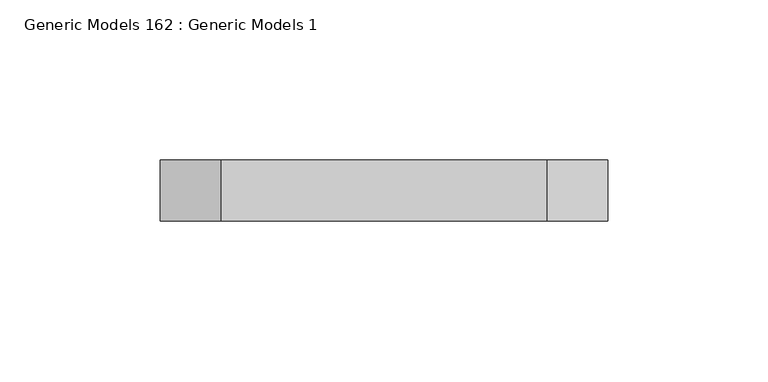
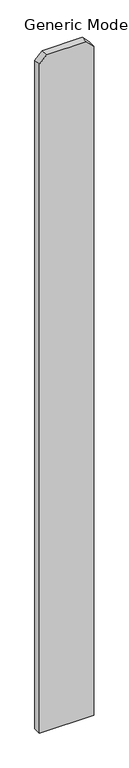
"""IFC4 building model written with IfcOpenShell, lengths in millimetres: proxy geometry, Generic Models 162 : Generic Models 1."""

import ifcopenshell
import ifcopenshell.guid

model = None  # the IFC model being written
_history = None  # IfcOwnerHistory: only IFC2X3 demands one
_inside = {}  # id of a spatial element -> (the spatial element, [elements in it])
_under = {}  # id of a project, library or spatial element -> (it, [spatial elements below it])
_declared = {}  # id of a project -> (the project, [libraries it declares])
_typed = {}  # id of a type object -> (the type object, [elements of that type])
_made_of = {}  # id of a material, layer set ... -> (it, [elements and type objects made of it])


def new_model(schema):
    """Start an empty IFC model of exactly this schema.

    Asked for "IFC4X3", IfcOpenShell would pick the latest addendum, in which some entities
    have other attributes; the version numbers below select the first issue.
    IFC2X3 requires an IfcOwnerHistory on every rooted entity: one is made here for all.
    """
    global model, _history
    if schema == "IFC4X3":
        model = ifcopenshell.file(schema_version=(4, 3, 0, 0))
    else:
        model = ifcopenshell.file(schema=schema)
    _inside.clear()
    _under.clear()
    _declared.clear()
    _typed.clear()
    _made_of.clear()
    _history = None
    if model.schema == "IFC2X3":
        org = make("IfcOrganization", Name="unknown")
        user = make(
            "IfcPersonAndOrganization",
            ThePerson=make("IfcPerson", FamilyName="unknown"),
            TheOrganization=org,
        )
        app = make(
            "IfcApplication",
            ApplicationDeveloper=org,
            Version="unknown",
            ApplicationFullName="unknown",
            ApplicationIdentifier="unknown",
        )
        _history = make(
            "IfcOwnerHistory",
            OwningUser=user,
            OwningApplication=app,
            ChangeAction="ADDED",
            CreationDate=0,
        )
    return model


def make(cls, **values):
    """One entity of the class cls with the attributes given. An attribute that is None is left unset."""
    return model.create_entity(
        cls, **{name: value for name, value in values.items() if value is not None}
    )


def rooted(cls, **values):
    """An entity with a GlobalId (a new one), such as an element, a storey or a relation."""
    return make(cls, GlobalId=ifcopenshell.guid.new(), OwnerHistory=_history, **values)


def si_unit(unit_type, name, prefix=None):
    """IfcSIUnit, for example si_unit("LENGTHUNIT", "METRE", prefix="MILLI")."""
    return make("IfcSIUnit", UnitType=unit_type, Prefix=prefix, Name=name)


def assignment(units):
    """IfcUnitAssignment: the units of a project."""
    return None if units is None else make("IfcUnitAssignment", Units=units)


def point(xyz):
    """IfcCartesianPoint."""
    return None if xyz is None else make("IfcCartesianPoint", Coordinates=xyz)


def direction(xyz):
    """IfcDirection."""
    return None if xyz is None else make("IfcDirection", DirectionRatios=xyz)


def frame(location, z_axis=None, x_axis=None):
    """IfcAxis2Placement3D, a coordinate frame: its origin and axes. An axis left out is left unset."""
    return make(
        "IfcAxis2Placement3D",
        Location=point(location),
        Axis=direction(z_axis),
        RefDirection=direction(x_axis),
    )


def origin():
    """The frame at (0, 0, 0) with its axes left unset."""
    return frame((0.0, 0.0, 0.0))


def place(relative_to, where):
    """IfcLocalPlacement: puts the frame where relative to a parent placement (None: the world)."""
    return make(
        "IfcLocalPlacement", PlacementRelTo=relative_to, RelativePlacement=where
    )


def context(
    kind, dimensions, precision=None, world=None, true_north=None, identifier=None
):
    """IfcGeometricRepresentationContext, for example the 3D "Model" context."""
    return make(
        "IfcGeometricRepresentationContext",
        ContextIdentifier=identifier,
        ContextType=kind,
        CoordinateSpaceDimension=dimensions,
        Precision=precision,
        WorldCoordinateSystem=world,
        TrueNorth=true_north,
    )


def project(units=None, contexts=None):
    """IfcProject with its units and contexts."""
    return rooted(
        "IfcProject",
        Name="project",
        RepresentationContexts=contexts,
        UnitsInContext=assignment(units),
    )


def spatial(cls, under=None, at=None, **own):
    """A site, building, storey or space (cls), placed at a placement, below another one or the project."""
    s = rooted(cls, ObjectPlacement=at, **own)
    if under is not None:
        _under.setdefault(under.id(), (under, []))[1].append(s)
    return s


def polyline(points):
    """IfcPolyline through the points."""
    return make("IfcPolyline", Points=[point(p) for p in points])


def outline(outer, holes=None, kind="AREA"):
    """IfcArbitraryClosedProfileDef: a profile drawn as a closed curve; with holes, ...WithVoids."""
    if holes is None:
        return make("IfcArbitraryClosedProfileDef", ProfileType=kind, OuterCurve=outer)
    return make(
        "IfcArbitraryProfileDefWithVoids",
        ProfileType=kind,
        OuterCurve=outer,
        InnerCurves=holes,
    )


def extrude(swept, where, along, depth):
    """IfcExtrudedAreaSolid: the profile swept, set in the frame where, extruded along a direction by depth."""
    return make(
        "IfcExtrudedAreaSolid",
        SweptArea=swept,
        Position=where,
        ExtrudedDirection=direction(along),
        Depth=depth,
    )


def shape(context_of_items, identifier, shape_type, items):
    """IfcShapeRepresentation: the items that make up one representation, for example the "Body"."""
    return make(
        "IfcShapeRepresentation",
        ContextOfItems=context_of_items,
        RepresentationIdentifier=identifier,
        RepresentationType=shape_type,
        Items=items,
    )


def source(mapping_origin, context_of_items, identifier, shape_type, items):
    """IfcRepresentationMap: a shape defined once, which mapped items show again and again."""
    return make(
        "IfcRepresentationMap",
        MappingOrigin=mapping_origin,
        MappedRepresentation=shape(context_of_items, identifier, shape_type, items),
    )


def transform(
    local_origin,
    x_axis=None,
    y_axis=None,
    z_axis=None,
    scale=None,
    scale2=None,
    scale3=None,
    uniform=True,
):
    """IfcCartesianTransformationOperator3D, or its non-uniform kind. x_axis, y_axis, z_axis: its Axis1, 2, 3."""
    if uniform:
        return make(
            "IfcCartesianTransformationOperator3D",
            Axis1=direction(x_axis),
            Axis2=direction(y_axis),
            LocalOrigin=point(local_origin),
            Scale=scale,
            Axis3=direction(z_axis),
        )
    return make(
        "IfcCartesianTransformationOperator3DnonUniform",
        Axis1=direction(x_axis),
        Axis2=direction(y_axis),
        LocalOrigin=point(local_origin),
        Scale=scale,
        Axis3=direction(z_axis),
        Scale2=scale2,
        Scale3=scale3,
    )


def mapped(mapping_source, mapping_target):
    """IfcMappedItem: shows the shape of a source again, moved by a transform."""
    return make(
        "IfcMappedItem", MappingSource=mapping_source, MappingTarget=mapping_target
    )


def made_of(thing, what):
    """Note that an element or type object is made of a material, layer set ...; save() writes the relation."""
    if what is not None:
        _made_of.setdefault(what.id(), (what, []))[1].append(thing)
    return thing


def element(
    cls,
    number,
    at=None,
    inside=None,
    cuts=None,
    type_object=None,
    material=None,
    context=None,
    identifier="Body",
    shape_type=None,
    held_by="IfcProductDefinitionShape",
    body=None,
    shapes=None,
    **own,
):
    """One element of the class cls, such as IfcWall. Its Tag is "e" and its number.

    at: its placement. inside: the storey or other place that contains it. cuts: it is an
    opening in that element (IfcRelVoidsElement). A single representation is given by context,
    identifier, shape_type and body (its items); several are given by shapes. held_by: the class
    of the entity that holds the representations. save() writes the other relations.
    """
    e = rooted(cls, Tag="e%d" % number, ObjectPlacement=at, **own)
    if body is not None:
        shapes = [shape(context, identifier, shape_type, body)]
    if shapes is not None:
        e.Representation = make(held_by, Representations=shapes)
    if inside is not None:
        _inside.setdefault(inside.id(), (inside, []))[1].append(e)
    if cuts is not None:
        rooted(
            "IfcRelVoidsElement", RelatingBuildingElement=cuts, RelatedOpeningElement=e
        )
    if type_object is not None:
        _typed.setdefault(type_object.id(), (type_object, []))[1].append(e)
    return made_of(e, material)


def aggregate(whole, parts):
    """IfcRelAggregates: a whole, such as a stair, and the parts it consists of."""
    return rooted("IfcRelAggregates", RelatingObject=whole, RelatedObjects=parts)


def save(model, path):
    """Write the relations noted so far, then the file.

    IfcRelAggregates (storeys below a building ...), IfcRelContainedInSpatialStructure (elements
    in a storey), IfcRelDefinesByType, IfcRelAssociatesMaterial and IfcRelDeclares: one each for
    every whole, place, type object, material and project.
    """
    for whole, parts in _under.values():
        aggregate(whole, parts)
    for where, things in _inside.values():
        rooted(
            "IfcRelContainedInSpatialStructure",
            RelatedElements=things,
            RelatingStructure=where,
        )
    for kind, things in _typed.values():
        rooted("IfcRelDefinesByType", RelatedObjects=things, RelatingType=kind)
    for what, things in _made_of.values():
        rooted("IfcRelAssociatesMaterial", RelatedObjects=things, RelatingMaterial=what)
    for by, libraries in _declared.values():
        rooted("IfcRelDeclares", RelatingContext=by, RelatedDefinitions=libraries)
    model.write(path)


def generic_models_162_generic_models_1_249433e1(model_context):
    return source(origin(), model_context, "Body", "SweptSolid", [
        extrude(outline(polyline([(76.2, 54684.6125), (1885.95, 54684.6125), (1905.0, 54665.5625), (1905.0, 54563.9625), (1885.95, 54544.9125), (76.2, 54544.9125), (76.2, 54684.6125)])), frame((0.0, 547.6875, 0.0), z_axis=(0.0, 1.0, 0.0), x_axis=(0.0, 0.0, 1.0)), (0.0, 0.0, 1.0), 19.05),
    ])


if __name__ == "__main__":
    model = new_model("IFC4")
    model_context = context("Model", 3, world=origin())
    ifc_project = project(units=[si_unit("LENGTHUNIT", "METRE", prefix="MILLI")], contexts=[model_context])
    site = spatial("IfcSite", under=ifc_project)
    building = spatial("IfcBuilding", under=site)
    placement = place(None, origin())
    generic_models_162_generic_models_1_shape = generic_models_162_generic_models_1_249433e1(model_context)
    element("IfcBuildingElementProxy", 1, Name="Generic Models 162 : Generic Models 1", ObjectType="Generic Models 162 : Generic Models 1", at=placement, inside=building, context=model_context, shape_type="MappedRepresentation", body=[
        mapped(generic_models_162_generic_models_1_shape, transform((0.0, 0.0, 0.0), x_axis=(1.0, 0.0, 0.0), y_axis=(0.0, 1.0, 0.0), z_axis=(0.0, 0.0, 1.0))),
    ])
    save(model, "model.ifc")

# Revit data of these elements
# Element 1 (IfcBuildingElementProxy, "Generic Models 162 : Generic Models 1")
#   Materials on its faces: "VERTICAL 1X6 CEDAR PLANKS W/ CLEAR WOOD SEALER"
# Materials
#   "VERTICAL 1X6 CEDAR PLANKS W/ CLEAR WOOD SEALER": class "Wood", colour RGB 234 198 147, transparency 0, Description = "Pinus Echinata", Cost = 0
